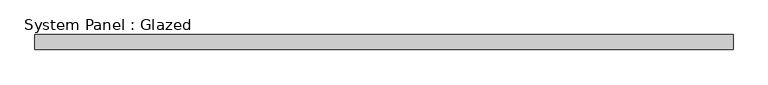
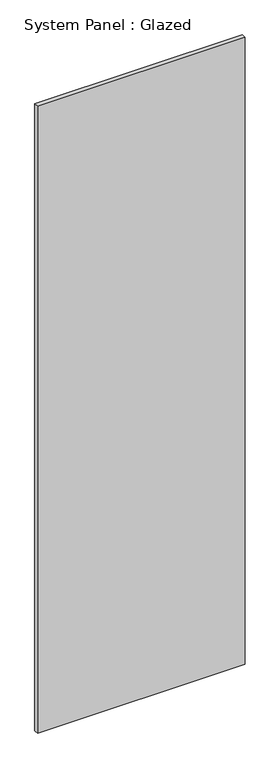
"""IFC4 building model written with IfcOpenShell, lengths in millimetres: plate geometry, System Panel : Glazed."""

import ifcopenshell
import ifcopenshell.guid

model = None  # the IFC model being written
_history = None  # IfcOwnerHistory: only IFC2X3 demands one
_inside = {}  # id of a spatial element -> (the spatial element, [elements in it])
_under = {}  # id of a project, library or spatial element -> (it, [spatial elements below it])
_declared = {}  # id of a project -> (the project, [libraries it declares])
_typed = {}  # id of a type object -> (the type object, [elements of that type])
_made_of = {}  # id of a material, layer set ... -> (it, [elements and type objects made of it])


def new_model(schema):
    """Start an empty IFC model of exactly this schema.

    Asked for "IFC4X3", IfcOpenShell would pick the latest addendum, in which some entities
    have other attributes; the version numbers below select the first issue.
    IFC2X3 requires an IfcOwnerHistory on every rooted entity: one is made here for all.
    """
    global model, _history
    if schema == "IFC4X3":
        model = ifcopenshell.file(schema_version=(4, 3, 0, 0))
    else:
        model = ifcopenshell.file(schema=schema)
    _inside.clear()
    _under.clear()
    _declared.clear()
    _typed.clear()
    _made_of.clear()
    _history = None
    if model.schema == "IFC2X3":
        org = make("IfcOrganization", Name="unknown")
        user = make(
            "IfcPersonAndOrganization",
            ThePerson=make("IfcPerson", FamilyName="unknown"),
            TheOrganization=org,
        )
        app = make(
            "IfcApplication",
            ApplicationDeveloper=org,
            Version="unknown",
            ApplicationFullName="unknown",
            ApplicationIdentifier="unknown",
        )
        _history = make(
            "IfcOwnerHistory",
            OwningUser=user,
            OwningApplication=app,
            ChangeAction="ADDED",
            CreationDate=0,
        )
    return model


def make(cls, **values):
    """One entity of the class cls with the attributes given. An attribute that is None is left unset."""
    return model.create_entity(
        cls, **{name: value for name, value in values.items() if value is not None}
    )


def rooted(cls, **values):
    """An entity with a GlobalId (a new one), such as an element, a storey or a relation."""
    return make(cls, GlobalId=ifcopenshell.guid.new(), OwnerHistory=_history, **values)


def si_unit(unit_type, name, prefix=None):
    """IfcSIUnit, for example si_unit("LENGTHUNIT", "METRE", prefix="MILLI")."""
    return make("IfcSIUnit", UnitType=unit_type, Prefix=prefix, Name=name)


def assignment(units):
    """IfcUnitAssignment: the units of a project."""
    return None if units is None else make("IfcUnitAssignment", Units=units)


def point(xyz):
    """IfcCartesianPoint."""
    return None if xyz is None else make("IfcCartesianPoint", Coordinates=xyz)


def direction(xyz):
    """IfcDirection."""
    return None if xyz is None else make("IfcDirection", DirectionRatios=xyz)


def frame(location, z_axis=None, x_axis=None):
    """IfcAxis2Placement3D, a coordinate frame: its origin and axes. An axis left out is left unset."""
    return make(
        "IfcAxis2Placement3D",
        Location=point(location),
        Axis=direction(z_axis),
        RefDirection=direction(x_axis),
    )


def origin():
    """The frame at (0, 0, 0) with its axes left unset."""
    return frame((0.0, 0.0, 0.0))


def origin_with_axes():
    """The frame at (0, 0, 0) with the z axis (0, 0, 1) and the x axis (1, 0, 0) written out."""
    return frame((0.0, 0.0, 0.0), z_axis=(0.0, 0.0, 1.0), x_axis=(1.0, 0.0, 0.0))


def place(relative_to, where):
    """IfcLocalPlacement: puts the frame where relative to a parent placement (None: the world)."""
    return make(
        "IfcLocalPlacement", PlacementRelTo=relative_to, RelativePlacement=where
    )


def context(
    kind, dimensions, precision=None, world=None, true_north=None, identifier=None
):
    """IfcGeometricRepresentationContext, for example the 3D "Model" context."""
    return make(
        "IfcGeometricRepresentationContext",
        ContextIdentifier=identifier,
        ContextType=kind,
        CoordinateSpaceDimension=dimensions,
        Precision=precision,
        WorldCoordinateSystem=world,
        TrueNorth=true_north,
    )


def project(units=None, contexts=None):
    """IfcProject with its units and contexts."""
    return rooted(
        "IfcProject",
        Name="project",
        RepresentationContexts=contexts,
        UnitsInContext=assignment(units),
    )


def spatial(cls, under=None, at=None, **own):
    """A site, building, storey or space (cls), placed at a placement, below another one or the project."""
    s = rooted(cls, ObjectPlacement=at, **own)
    if under is not None:
        _under.setdefault(under.id(), (under, []))[1].append(s)
    return s


def polyline(points):
    """IfcPolyline through the points."""
    return make("IfcPolyline", Points=[point(p) for p in points])


def outline(outer, holes=None, kind="AREA"):
    """IfcArbitraryClosedProfileDef: a profile drawn as a closed curve; with holes, ...WithVoids."""
    if holes is None:
        return make("IfcArbitraryClosedProfileDef", ProfileType=kind, OuterCurve=outer)
    return make(
        "IfcArbitraryProfileDefWithVoids",
        ProfileType=kind,
        OuterCurve=outer,
        InnerCurves=holes,
    )


def extrude(swept, where, along, depth):
    """IfcExtrudedAreaSolid: the profile swept, set in the frame where, extruded along a direction by depth."""
    return make(
        "IfcExtrudedAreaSolid",
        SweptArea=swept,
        Position=where,
        ExtrudedDirection=direction(along),
        Depth=depth,
    )


def shape(context_of_items, identifier, shape_type, items):
    """IfcShapeRepresentation: the items that make up one representation, for example the "Body"."""
    return make(
        "IfcShapeRepresentation",
        ContextOfItems=context_of_items,
        RepresentationIdentifier=identifier,
        RepresentationType=shape_type,
        Items=items,
    )


def source(mapping_origin, context_of_items, identifier, shape_type, items):
    """IfcRepresentationMap: a shape defined once, which mapped items show again and again."""
    return make(
        "IfcRepresentationMap",
        MappingOrigin=mapping_origin,
        MappedRepresentation=shape(context_of_items, identifier, shape_type, items),
    )


def transform(
    local_origin,
    x_axis=None,
    y_axis=None,
    z_axis=None,
    scale=None,
    scale2=None,
    scale3=None,
    uniform=True,
):
    """IfcCartesianTransformationOperator3D, or its non-uniform kind. x_axis, y_axis, z_axis: its Axis1, 2, 3."""
    if uniform:
        return make(
            "IfcCartesianTransformationOperator3D",
            Axis1=direction(x_axis),
            Axis2=direction(y_axis),
            LocalOrigin=point(local_origin),
            Scale=scale,
            Axis3=direction(z_axis),
        )
    return make(
        "IfcCartesianTransformationOperator3DnonUniform",
        Axis1=direction(x_axis),
        Axis2=direction(y_axis),
        LocalOrigin=point(local_origin),
        Scale=scale,
        Axis3=direction(z_axis),
        Scale2=scale2,
        Scale3=scale3,
    )


def mapped(mapping_source, mapping_target):
    """IfcMappedItem: shows the shape of a source again, moved by a transform."""
    return make(
        "IfcMappedItem", MappingSource=mapping_source, MappingTarget=mapping_target
    )


def made_of(thing, what):
    """Note that an element or type object is made of a material, layer set ...; save() writes the relation."""
    if what is not None:
        _made_of.setdefault(what.id(), (what, []))[1].append(thing)
    return thing


def element(
    cls,
    number,
    at=None,
    inside=None,
    cuts=None,
    type_object=None,
    material=None,
    context=None,
    identifier="Body",
    shape_type=None,
    held_by="IfcProductDefinitionShape",
    body=None,
    shapes=None,
    **own,
):
    """One element of the class cls, such as IfcWall. Its Tag is "e" and its number.

    at: its placement. inside: the storey or other place that contains it. cuts: it is an
    opening in that element (IfcRelVoidsElement). A single representation is given by context,
    identifier, shape_type and body (its items); several are given by shapes. held_by: the class
    of the entity that holds the representations. save() writes the other relations.
    """
    e = rooted(cls, Tag="e%d" % number, ObjectPlacement=at, **own)
    if body is not None:
        shapes = [shape(context, identifier, shape_type, body)]
    if shapes is not None:
        e.Representation = make(held_by, Representations=shapes)
    if inside is not None:
        _inside.setdefault(inside.id(), (inside, []))[1].append(e)
    if cuts is not None:
        rooted(
            "IfcRelVoidsElement", RelatingBuildingElement=cuts, RelatedOpeningElement=e
        )
    if type_object is not None:
        _typed.setdefault(type_object.id(), (type_object, []))[1].append(e)
    return made_of(e, material)


def aggregate(whole, parts):
    """IfcRelAggregates: a whole, such as a stair, and the parts it consists of."""
    return rooted("IfcRelAggregates", RelatingObject=whole, RelatedObjects=parts)


def save(model, path):
    """Write the relations noted so far, then the file.

    IfcRelAggregates (storeys below a building ...), IfcRelContainedInSpatialStructure (elements
    in a storey), IfcRelDefinesByType, IfcRelAssociatesMaterial and IfcRelDeclares: one each for
    every whole, place, type object, material and project.
    """
    for whole, parts in _under.values():
        aggregate(whole, parts)
    for where, things in _inside.values():
        rooted(
            "IfcRelContainedInSpatialStructure",
            RelatedElements=things,
            RelatingStructure=where,
        )
    for kind, things in _typed.values():
        rooted("IfcRelDefinesByType", RelatedObjects=things, RelatingType=kind)
    for what, things in _made_of.values():
        rooted("IfcRelAssociatesMaterial", RelatedObjects=things, RelatingMaterial=what)
    for by, libraries in _declared.values():
        rooted("IfcRelDeclares", RelatingContext=by, RelatedDefinitions=libraries)
    model.write(path)


def system_panel_glazed_4a693619(model_context):
    return source(origin(), model_context, "Body", "SweptSolid", [
        extrude(outline(polyline([(587.8744819, 19.05), (-587.8744819, 19.05), (-587.8744819, 44.45), (587.8744819, 44.45), (587.8744819, 19.05)])), origin_with_axes(), (0.0, 0.0, 1.0), 3746.5),
    ])


if __name__ == "__main__":
    model = new_model("IFC4")
    model_context = context("Model", 3, world=origin())
    ifc_project = project(units=[si_unit("LENGTHUNIT", "METRE", prefix="MILLI")], contexts=[model_context])
    site = spatial("IfcSite", under=ifc_project)
    building = spatial("IfcBuilding", under=site)
    placement = place(None, origin())
    system_panel_glazed_shape = system_panel_glazed_4a693619(model_context)
    element("IfcPlate", 1, ObjectType="System Panel : Glazed", at=placement, inside=building, context=model_context, shape_type="MappedRepresentation", body=[
        mapped(system_panel_glazed_shape, transform((0.0, 0.0, 0.0), x_axis=(1.0, 0.0, 0.0), y_axis=(0.0, 1.0, 0.0), z_axis=(0.0, 0.0, 1.0))),
    ])
    save(model, "model.ifc")

# Revit data of these elements
# Type "System Panel : Glazed"
#   Construction Type Id = "GSP4R"
#   Analytic Construction = "1/8 in Pilkington single glazing"
#   Visual Light Transmittance = 0.9
#   Solar Heat Gain Coefficient = 0.86
#   Heat Transfer Coefficient (U) = 1.18115 BTU/(h·ft²·°F)
#   Define Thermal Properties by = 1
# Element 1 (IfcPlate, "System Panel : Glazed")
#   Materials on its faces: "Glass"
# Materials
#   "Glass": class "Glass", colour RGB 0 128 192, transparency 0.75, Description = "Soda Lime Glass", Cost = 0
